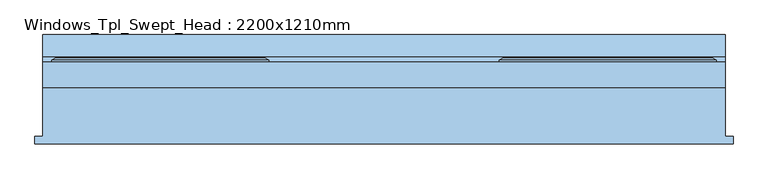
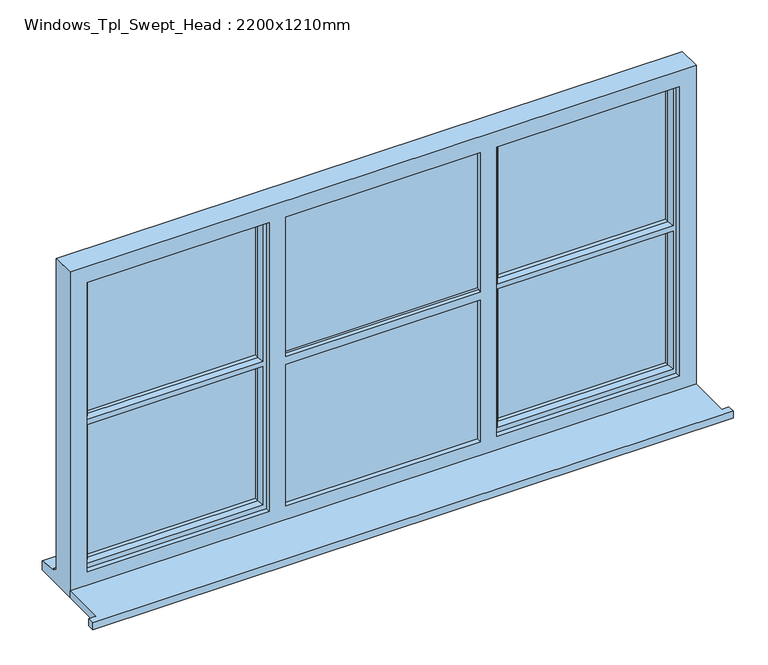
"""IFC4 building model written with IfcOpenShell, lengths in millimetres: window geometry, Windows_Tpl_Swept_Head : 2200x1210mm."""

from ifc_helpers import new_model, si_unit, point, frame, frame_2d, origin, place, context, project, spatial, polyline, circle_curve, trimmed, segment, composite_curve, outline, extrude, faceted_brep, source, transform, mapped, element, save


def windows_tpl_swept_head_2200x1210mm_9d782c46(model_context):
    return source(origin(), model_context, "Body", "SolidModel", [
        extrude(outline(polyline([(-1766.6666667, -161.5434322), (-1766.6666667, -136.5434322), (-1741.6666667, -136.5434322), (-1741.6666667, 20.4565678), (458.3333333, 20.4565678), (458.3333333, -136.5434322), (483.3333333, -136.5434322), (483.3333333, -161.5434322), (-1766.6666667, -161.5434322)])), frame((0.0, 0.0, 900.0), z_axis=(0.0, 0.0, 1.0), x_axis=(1.0, 0.0, 0.0)), (0.0, 0.0, 1.0), 25.0),
        extrude(outline(composite_curve([segment(polyline([(2050.0, -300.0), (2050.0, -983.3333333), (1935.9532624, -983.3333333)]), True, "CONTINUOUS"), segment(trimmed(circle_curve(frame_2d((1325.0, -641.6666667)), 700.0), [point((1935.9532624, -983.3333333))], [point((1935.9532624, -300.0))], True, "CARTESIAN"), True, "CONTINUOUS"), segment(polyline([(1935.9532624, -300.0), (2050.0, -300.0)]), True, "CONTINUOUS")], self_intersect=False)), frame((0.0, 62.4565678, 0.0), z_axis=(0.0, 1.0, 0.0), x_axis=(0.0, 0.0, 1.0)), (0.0, 0.0, 1.0), 25.0),
        extrude(outline(composite_curve([segment(polyline([(2030.0, -220.0), (1957.8501446, -220.0)]), True, "CONTINUOUS"), segment(trimmed(circle_curve(frame_2d((1325.0, 79.1666667)), 700.0), [point((1957.8501446, -220.0))], [point((1957.8501446, 378.3333333))], True, "CARTESIAN"), True, "CONTINUOUS"), segment(polyline([(1957.8501446, 378.3333333), (2030.0, 378.3333333), (2030.0, -220.0)]), True, "CONTINUOUS")], self_intersect=False)), frame((0.0, 79.4565678, 0.0), z_axis=(0.0, 1.0, 0.0), x_axis=(0.0, 0.0, 1.0)), (0.0, 0.0, 1.0), 24.0),
        extrude(outline(composite_curve([segment(polyline([(2030.0, -1063.3333333), (2030.0, -1661.6666667), (1957.8501446, -1661.6666667)]), True, "CONTINUOUS"), segment(trimmed(circle_curve(frame_2d((1325.0, -1362.5)), 700.0), [point((1957.8501446, -1661.6666667))], [point((1957.8501446, -1063.3333333))], True, "CARTESIAN"), True, "CONTINUOUS"), segment(polyline([(1957.8501446, -1063.3333333), (2030.0, -1063.3333333)]), True, "CONTINUOUS")], self_intersect=False)), frame((0.0, 79.4565678, 0.0), z_axis=(0.0, 1.0, 0.0), x_axis=(0.0, 0.0, 1.0)), (0.0, 0.0, 1.0), 24.0),
        faceted_brep([(-270.0, 103.4565678, 2080.0), (-270.0, 109.2300705, 2080.0), (-270.0, 109.2300705, 953.0), (-270.0, 103.4565678, 953.0), (-260.0, 38.4565678, 2070.0), (-260.0, 103.4565678, 2070.0), (-260.0, 103.4565678, 963.0), (-260.0, 38.4565678, 963.0), (-220.0, 52.9494677, 2030.0), (-230.1480377, 38.4565678, 2040.1480377), (-230.1480377, 38.4565678, 1526.3519623), (-220.0, 52.9494677, 1536.5), (-230.1480377, 38.4565678, 992.8519623), (-220.0, 52.9494677, 1003.0), (-220.0, 52.9494677, 1496.5), (-230.1480377, 38.4565678, 1506.6480377), (-220.0, 67.4565678, 2030.0), (-220.0, 67.4565678, 1536.5), (-220.0, 67.4565678, 1003.0), (-220.0, 67.4565678, 1496.5), (-230.0, 91.4565678, 1529.5), (-230.0, 91.4565678, 2040.0), (-230.0, 67.4565678, 2040.0), (-230.0, 67.4565678, 1529.5), (-230.0, 67.4565678, 1503.5), (-230.0, 67.4565678, 993.0), (-230.0, 91.4565678, 993.0), (-230.0, 91.4565678, 1503.5), (-220.0, 109.2300705, 2030.0), (-220.0, 91.4565678, 2030.0), (-220.0, 91.4565678, 1536.5), (-220.0, 109.2300705, 1536.5), (-220.0, 91.4565678, 1003.0), (-220.0, 109.2300705, 1003.0), (-220.0, 109.2300705, 1496.5), (-220.0, 91.4565678, 1496.5), (-237.4457548, 115.0035732, 2047.4457548), (-237.4457548, 115.0035732, 1519.0542452), (-237.4457548, 115.0035732, 985.5542452), (-237.4457548, 115.0035732, 1513.9457548), (-259.2153903, 115.0035732, 2069.2153903), (-259.2153903, 115.0035732, 963.7846097), (428.3333333, 109.2300705, 953.0), (428.3333333, 103.4565678, 953.0), (418.3333333, 103.4565678, 963.0), (418.3333333, 38.4565678, 963.0), (388.4813711, 38.4565678, 992.8519623), (378.3333333, 52.9494677, 1003.0), (378.3333333, 67.4565678, 1003.0), (388.3333333, 67.4565678, 993.0), (388.3333333, 91.4565678, 993.0), (378.3333333, 91.4565678, 1003.0), (378.3333333, 109.2300705, 1003.0), (395.7790881, 115.0035732, 985.5542452), (417.5487236, 115.0035732, 963.7846097), (428.3333333, 109.2300705, 2080.0), (428.3333333, 103.4565678, 2080.0), (418.3333333, 103.4565678, 2070.0), (418.3333333, 38.4565678, 2070.0), (388.4813711, 38.4565678, 1506.6480377), (378.3333333, 52.9494677, 1496.5), (388.4813711, 38.4565678, 2040.1480377), (378.3333333, 52.9494677, 2030.0), (378.3333333, 52.9494677, 1536.5), (388.4813711, 38.4565678, 1526.3519623), (378.3333333, 67.4565678, 1496.5), (378.3333333, 67.4565678, 2030.0), (378.3333333, 67.4565678, 1536.5), (388.3333333, 91.4565678, 1503.5), (388.3333333, 67.4565678, 1503.5), (388.3333333, 67.4565678, 1529.5), (388.3333333, 67.4565678, 2040.0), (388.3333333, 91.4565678, 2040.0), (388.3333333, 91.4565678, 1529.5), (378.3333333, 91.4565678, 1496.5), (378.3333333, 109.2300705, 1496.5), (378.3333333, 91.4565678, 2030.0), (378.3333333, 109.2300705, 2030.0), (378.3333333, 109.2300705, 1536.5), (378.3333333, 91.4565678, 1536.5), (395.7790881, 115.0035732, 1513.9457548), (395.7790881, 115.0035732, 2047.4457548), (395.7790881, 115.0035732, 1519.0542452), (417.5487236, 115.0035732, 2069.2153903)], [[[0, 1, 2, 3]], [[4, 5, 6, 7]], [[8, 9, 10, 11]], [[12, 13, 14, 15]], [[16, 8, 11, 17]], [[13, 18, 19, 14]], [[20, 21, 22, 23]], [[24, 25, 26, 27]], [[28, 29, 30, 31]], [[32, 33, 34, 35]], [[36, 28, 31, 37]], [[33, 38, 39, 34]], [[2, 1, 40, 41]], [[3, 2, 42, 43]], [[7, 6, 44, 45]], [[13, 12, 46, 47]], [[18, 13, 47, 48]], [[26, 25, 49, 50]], [[33, 32, 51, 52]], [[38, 33, 52, 53]], [[2, 41, 54, 42]], [[43, 42, 55, 56]], [[45, 44, 57, 58]], [[47, 46, 59, 60]], [[61, 62, 63, 64]], [[48, 47, 60, 65]], [[62, 66, 67, 63]], [[68, 50, 49, 69]], [[70, 71, 72, 73]], [[52, 51, 74, 75]], [[76, 77, 78, 79]], [[53, 52, 75, 80]], [[77, 81, 82, 78]], [[42, 54, 83, 55]], [[1, 0, 56, 55]], [[0, 3, 43, 56], [6, 5, 57, 44]], [[5, 4, 58, 57]], [[4, 7, 45, 58], [46, 12, 15, 59], [61, 64, 10, 9]], [[9, 8, 62, 61]], [[8, 16, 66, 62]], [[49, 25, 24, 69], [18, 48, 65, 19]], [[22, 71, 70, 23], [66, 16, 17, 67]], [[22, 21, 72, 71]], [[26, 50, 68, 27], [32, 35, 74, 51]], [[72, 21, 20, 73], [76, 79, 30, 29]], [[29, 28, 77, 76]], [[28, 36, 81, 77]], [[41, 40, 83, 54], [36, 37, 82, 81], [38, 53, 80, 39]], [[40, 1, 55, 83]], [[82, 37, 31, 78]], [[30, 79, 78, 31]], [[73, 20, 23, 70]], [[11, 63, 67, 17]], [[10, 64, 63, 11]], [[59, 15, 14, 60]], [[60, 14, 19, 65]], [[27, 68, 69, 24]], [[74, 35, 34, 75]], [[39, 80, 75, 34]]]),
        faceted_brep([(-1013.3333333, 103.4565678, 2080.0), (-1013.3333333, 109.2300705, 2080.0), (-1711.6666667, 109.2300705, 2080.0), (-1711.6666667, 103.4565678, 2080.0), (-1023.3333333, 38.4565678, 2070.0), (-1023.3333333, 103.4565678, 2070.0), (-1701.6666667, 103.4565678, 2070.0), (-1701.6666667, 38.4565678, 2070.0), (-1063.3333333, 52.9494677, 2030.0), (-1053.1852956, 38.4565678, 2040.1480377), (-1671.8147044, 38.4565678, 2040.1480377), (-1661.6666667, 52.9494677, 2030.0), (-1661.6666667, 67.4565678, 2030.0), (-1063.3333333, 67.4565678, 2030.0), (-1053.3333333, 91.4565678, 2040.0), (-1053.3333333, 67.4565678, 2040.0), (-1671.6666667, 67.4565678, 2040.0), (-1671.6666667, 91.4565678, 2040.0), (-1063.3333333, 109.2300705, 2030.0), (-1063.3333333, 91.4565678, 2030.0), (-1661.6666667, 91.4565678, 2030.0), (-1661.6666667, 109.2300705, 2030.0), (-1679.1124215, 115.0035732, 2047.4457548), (-1045.8875785, 115.0035732, 2047.4457548), (-1024.117943, 115.0035732, 2069.2153903), (-1700.882057, 115.0035732, 2069.2153903), (-1711.6666667, 109.2300705, 953.0), (-1711.6666667, 103.4565678, 953.0), (-1701.6666667, 103.4565678, 963.0), (-1701.6666667, 38.4565678, 963.0), (-1671.8147044, 38.4565678, 1526.3519623), (-1661.6666667, 52.9494677, 1536.5), (-1671.8147044, 38.4565678, 992.8519623), (-1661.6666667, 52.9494677, 1003.0), (-1661.6666667, 52.9494677, 1496.5), (-1671.8147044, 38.4565678, 1506.6480377), (-1661.6666667, 67.4565678, 1536.5), (-1661.6666667, 67.4565678, 1003.0), (-1661.6666667, 67.4565678, 1496.5), (-1671.6666667, 91.4565678, 1529.5), (-1671.6666667, 67.4565678, 1529.5), (-1671.6666667, 67.4565678, 1503.5), (-1671.6666667, 67.4565678, 993.0), (-1671.6666667, 91.4565678, 993.0), (-1671.6666667, 91.4565678, 1503.5), (-1661.6666667, 91.4565678, 1536.5), (-1661.6666667, 109.2300705, 1536.5), (-1661.6666667, 91.4565678, 1003.0), (-1661.6666667, 109.2300705, 1003.0), (-1661.6666667, 109.2300705, 1496.5), (-1661.6666667, 91.4565678, 1496.5), (-1679.1124215, 115.0035732, 1519.0542452), (-1679.1124215, 115.0035732, 985.5542452), (-1679.1124215, 115.0035732, 1513.9457548), (-1700.882057, 115.0035732, 963.7846097), (-1013.3333333, 109.2300705, 953.0), (-1013.3333333, 103.4565678, 953.0), (-1023.3333333, 103.4565678, 963.0), (-1023.3333333, 38.4565678, 963.0), (-1053.1852956, 38.4565678, 1526.3519623), (-1053.1852956, 38.4565678, 1506.6480377), (-1053.1852956, 38.4565678, 992.8519623), (-1063.3333333, 52.9494677, 1003.0), (-1063.3333333, 67.4565678, 1003.0), (-1053.3333333, 67.4565678, 1529.5), (-1063.3333333, 67.4565678, 1536.5), (-1053.3333333, 67.4565678, 993.0), (-1053.3333333, 67.4565678, 1503.5), (-1063.3333333, 67.4565678, 1496.5), (-1053.3333333, 91.4565678, 993.0), (-1053.3333333, 91.4565678, 1529.5), (-1063.3333333, 91.4565678, 1536.5), (-1053.3333333, 91.4565678, 1503.5), (-1063.3333333, 91.4565678, 1496.5), (-1063.3333333, 91.4565678, 1003.0), (-1063.3333333, 109.2300705, 1003.0), (-1045.8875785, 115.0035732, 985.5542452), (-1024.117943, 115.0035732, 963.7846097), (-1045.8875785, 115.0035732, 1519.0542452), (-1045.8875785, 115.0035732, 1513.9457548), (-1063.3333333, 52.9494677, 1536.5), (-1063.3333333, 52.9494677, 1496.5), (-1063.3333333, 109.2300705, 1536.5), (-1063.3333333, 109.2300705, 1496.5)], [[[0, 1, 2, 3]], [[4, 5, 6, 7]], [[8, 9, 10, 11]], [[8, 11, 12, 13]], [[14, 15, 16, 17]], [[18, 19, 20, 21]], [[18, 21, 22, 23]], [[2, 1, 24, 25]], [[3, 2, 26, 27]], [[7, 6, 28, 29]], [[11, 10, 30, 31]], [[32, 33, 34, 35]], [[12, 11, 31, 36]], [[33, 37, 38, 34]], [[39, 17, 16, 40]], [[41, 42, 43, 44]], [[21, 20, 45, 46]], [[47, 48, 49, 50]], [[22, 21, 46, 51]], [[48, 52, 53, 49]], [[2, 25, 54, 26]], [[27, 26, 55, 56]], [[0, 3, 27, 56], [6, 5, 57, 28]], [[29, 28, 57, 58]], [[4, 7, 29, 58], [10, 9, 59, 30], [32, 35, 60, 61]], [[33, 32, 61, 62]], [[37, 33, 62, 63]], [[16, 15, 64, 40], [13, 12, 36, 65]], [[66, 42, 41, 67], [37, 63, 68, 38]], [[43, 42, 66, 69]], [[14, 17, 39, 70], [19, 71, 45, 20]], [[43, 69, 72, 44], [47, 50, 73, 74]], [[48, 47, 74, 75]], [[52, 48, 75, 76]], [[25, 24, 77, 54], [23, 22, 51, 78], [76, 79, 53, 52]], [[26, 54, 77, 55]], [[1, 0, 56, 55]], [[5, 4, 58, 57]], [[9, 8, 80, 59]], [[62, 61, 60, 81]], [[8, 13, 65, 80]], [[63, 62, 81, 68]], [[64, 15, 14, 70]], [[72, 69, 66, 67]], [[19, 18, 82, 71]], [[75, 74, 73, 83]], [[18, 23, 78, 82]], [[76, 75, 83, 79]], [[24, 1, 55, 77]], [[78, 51, 46, 82]], [[45, 71, 82, 46]], [[40, 64, 70, 39]], [[65, 36, 31, 80]], [[30, 59, 80, 31]], [[60, 35, 34, 81]], [[38, 68, 81, 34]], [[67, 41, 44, 72]], [[73, 50, 49, 83]], [[53, 79, 83, 49]]]),
        extrude(outline(polyline([(388.4813711, 67.4565678), (-230.0, 67.4565678), (-230.0, 91.4565678), (388.4813711, 91.4565678), (388.4813711, 67.4565678)])), frame((0.0, 0.0, 993.0), z_axis=(0.0, 0.0, 1.0), x_axis=(1.0, 0.0, 0.0)), (0.0, 0.0, 1.0), 513.6480377),
        extrude(outline(polyline([(388.4813711, 67.4565678), (-230.0, 67.4565678), (-230.0, 91.4565678), (388.4813711, 91.4565678), (388.4813711, 67.4565678)])), frame((0.0, 0.0, 1526.3519623), z_axis=(0.0, 0.0, 1.0), x_axis=(1.0, 0.0, 0.0)), (0.0, 0.0, 1.0), 513.6480377),
        extrude(outline(polyline([(-993.3333333, 62.4565678), (-290.0, 62.4565678), (-290.0, 38.4565678), (-993.3333333, 38.4565678), (-993.3333333, 62.4565678)])), frame((0.0, 0.0, 963.0), z_axis=(0.0, 0.0, 1.0), x_axis=(1.0, 0.0, 0.0)), (0.0, 0.0, 1.0), 540.5),
        extrude(outline(polyline([(-993.3333333, 62.4565678), (-290.0, 62.4565678), (-290.0, 38.4565678), (-993.3333333, 38.4565678), (-993.3333333, 62.4565678)])), frame((0.0, 0.0, 1529.5), z_axis=(0.0, 0.0, 1.0), x_axis=(1.0, 0.0, 0.0)), (0.0, 0.0, 1.0), 540.5),
        extrude(outline(polyline([(-1053.3333333, 67.4565678), (-1671.6666667, 67.4565678), (-1671.6666667, 91.4565678), (-1053.3333333, 91.4565678), (-1053.3333333, 67.4565678)])), frame((0.0, 0.0, 1526.3519623), z_axis=(0.0, 0.0, 1.0), x_axis=(1.0, 0.0, 0.0)), (0.0, 0.0, 1.0), 513.6480377),
        extrude(outline(polyline([(-1053.3333333, 67.4565678), (-1671.6666667, 67.4565678), (-1671.6666667, 91.4565678), (-1053.3333333, 91.4565678), (-1053.3333333, 67.4565678)])), frame((0.0, 0.0, 993.0), z_axis=(0.0, 0.0, 1.0), x_axis=(1.0, 0.0, 0.0)), (0.0, 0.0, 1.0), 513.6480377),
        faceted_brep([(-983.3333333, 38.4565678, 2050.0), (-983.3333333, 20.4565678, 2050.0), (-983.3333333, 20.4565678, 1530.8390708), (-983.3333333, 28.5412125, 1536.5), (-983.3333333, 38.4565678, 1536.5), (-983.3333333, 20.4565678, 975.0), (-983.3333333, 38.4565678, 975.0), (-983.3333333, 38.4565678, 1496.5), (-983.3333333, 28.5412125, 1496.5), (-983.3333333, 20.4565678, 1502.1609292), (458.3333333, 20.4565678, 2110.0), (-1741.6666667, 20.4565678, 2110.0), (-1741.6666667, 20.4565678, 900.0), (458.3333333, 20.4565678, 900.0), (-1681.6666667, 20.4565678, 2050.0), (-1041.3333333, 20.4565678, 2050.0), (-1041.3333333, 20.4565678, 975.0), (-1681.6666667, 20.4565678, 975.0), (-242.0, 20.4565678, 2050.0), (398.3333333, 20.4565678, 2050.0), (398.3333333, 20.4565678, 975.0), (-242.0, 20.4565678, 975.0), (-300.0, 20.4565678, 2050.0), (-300.0, 20.4565678, 1530.8390708), (-300.0, 20.4565678, 975.0), (-300.0, 20.4565678, 1502.1609292), (-1041.3333333, 38.4565678, 2050.0), (-1041.3333333, 38.4565678, 975.0), (-1701.6666667, 38.4565678, 2070.0), (-1023.3333333, 38.4565678, 2070.0), (-1023.3333333, 38.4565678, 963.0), (-1701.6666667, 38.4565678, 963.0), (-1681.6666667, 38.4565678, 2050.0), (-1681.6666667, 38.4565678, 975.0), (-993.3333333, 38.4565678, 2070.0), (-290.0, 38.4565678, 2070.0), (-290.0, 38.4565678, 1529.5), (-983.3333333, 38.4565678, 1529.5), (-983.3333333, 38.4565678, 1503.5), (-290.0, 38.4565678, 1503.5), (-290.0, 38.4565678, 963.0), (-993.3333333, 38.4565678, 963.0), (-300.0, 38.4565678, 2050.0), (-300.0, 38.4565678, 1536.5), (-300.0, 38.4565678, 975.0), (-300.0, 38.4565678, 1496.5), (-260.0, 38.4565678, 2070.0), (418.3333333, 38.4565678, 2070.0), (418.3333333, 38.4565678, 963.0), (-260.0, 38.4565678, 963.0), (398.3333333, 38.4565678, 2050.0), (-242.0, 38.4565678, 2050.0), (-242.0, 38.4565678, 975.0), (398.3333333, 38.4565678, 975.0), (-1023.3333333, 103.4565678, 2070.0), (-1023.3333333, 103.4565678, 963.0), (-1741.6666667, 103.4565678, 2110.0), (458.3333333, 103.4565678, 2110.0), (458.3333333, 103.4565678, 951.0), (-1741.6666667, 103.4565678, 951.0), (-1701.6666667, 103.4565678, 2070.0), (-1701.6666667, 103.4565678, 963.0), (-983.3333333, 103.4565678, 2070.0), (-983.3333333, 103.4565678, 963.0), (-300.0, 103.4565678, 963.0), (-300.0, 103.4565678, 2070.0), (418.3333333, 103.4565678, 963.0), (418.3333333, 103.4565678, 2070.0), (-260.0, 103.4565678, 2070.0), (-260.0, 103.4565678, 963.0), (-983.3333333, 98.4565678, 2070.0), (-983.3333333, 98.4565678, 2050.0), (-983.3333333, 62.4565678, 2050.0), (-983.3333333, 62.4565678, 1536.5), (-983.3333333, 80.2300705, 1536.5), (-983.3333333, 86.0035732, 1519.0542452), (-983.3333333, 86.0035732, 1513.9457548), (-983.3333333, 80.2300705, 1496.5), (-983.3333333, 62.4565678, 1496.5), (-983.3333333, 62.4565678, 975.0), (-983.3333333, 98.4565678, 975.0), (-983.3333333, 98.4565678, 963.0), (-290.0, 62.4565678, 1503.5), (-983.3333333, 62.4565678, 1503.5), (-983.3333333, 62.4565678, 1529.5), (-290.0, 62.4565678, 1529.5), (-290.0, 62.4565678, 2070.0), (-993.3333333, 62.4565678, 2070.0), (-993.3333333, 62.4565678, 963.0), (-290.0, 62.4565678, 963.0), (-300.0, 62.4565678, 2050.0), (-300.0, 62.4565678, 1536.5), (-300.0, 62.4565678, 1496.5), (-300.0, 62.4565678, 975.0), (-1741.6666667, 118.4565678, 949.68767), (-1741.6666667, 118.4565678, 944.7449676), (-1741.6666667, 190.9565678, 933.8088847), (-1741.6666667, 190.9565678, 900.0), (-300.0, 98.4565678, 2070.0), (458.3333333, 190.9565678, 900.0), (458.3333333, 190.9565678, 933.8088847), (458.3333333, 118.4565678, 944.7449676), (458.3333333, 118.4565678, 949.68767), (-300.0, 98.4565678, 963.0), (-300.0, 98.4565678, 975.0), (-300.0, 80.2300705, 1496.5), (-300.0, 86.0035732, 1513.9457548), (-300.0, 86.0035732, 1519.0542452), (-300.0, 80.2300705, 1536.5), (-300.0, 98.4565678, 2050.0), (-300.0, 28.5412125, 1536.5), (-300.0, 28.5412125, 1496.5)], [[[0, 1, 2, 3, 4]], [[5, 6, 7, 8, 9]], [[10, 11, 12, 13], [14, 15, 16, 17], [18, 19, 20, 21], [1, 22, 23, 2], [24, 5, 9, 25]], [[15, 26, 27, 16]], [[28, 29, 30, 31], [26, 32, 33, 27]], [[34, 35, 36, 37, 38, 39, 40, 41], [42, 0, 4, 43], [6, 44, 45, 7]], [[46, 47, 48, 49], [50, 51, 52, 53]], [[54, 55, 30, 29]], [[56, 57, 58, 59], [55, 54, 60, 61], [62, 63, 64, 65], [66, 67, 68, 69]], [[63, 62, 70, 71, 72, 73, 74, 75, 76, 77, 78, 79, 80, 81]], [[82, 83, 84, 85, 86, 87, 88, 89], [73, 72, 90, 91], [92, 93, 79, 78]], [[88, 87, 34, 41]], [[11, 56, 59, 94, 95, 96, 97, 12]], [[61, 60, 28, 31]], [[32, 14, 17, 33]], [[11, 10, 57, 56]], [[62, 65, 98, 70]], [[87, 86, 35, 34]], [[28, 60, 54, 29]], [[67, 47, 46, 68]], [[1, 0, 42, 22]], [[14, 32, 26, 15]], [[50, 19, 18, 51]], [[57, 10, 13, 99, 100, 101, 102, 58]], [[67, 66, 48, 47]], [[19, 50, 53, 20]], [[82, 89, 40, 39]], [[35, 86, 85, 36]], [[65, 64, 103, 104, 93, 92, 105, 106, 107, 108, 91, 90, 109, 98]], [[69, 68, 46, 49]], [[51, 18, 21, 52]], [[22, 42, 43, 110, 23]], [[44, 24, 25, 111, 45]], [[99, 13, 12, 97]], [[100, 99, 97, 96]], [[101, 100, 96, 95]], [[102, 101, 95, 94]], [[58, 102, 94, 59]], [[55, 61, 31, 30]], [[64, 63, 81, 103]], [[66, 69, 49, 48]], [[89, 88, 41, 40]], [[17, 16, 27, 33]], [[21, 20, 53, 52]], [[44, 6, 5, 24]], [[83, 38, 37, 84]], [[75, 107, 106, 76]], [[76, 106, 105, 77]], [[92, 78, 77, 105]], [[38, 83, 82, 39]], [[7, 45, 111, 8]], [[25, 9, 8, 111]], [[2, 23, 110, 3]], [[43, 4, 3, 110]], [[84, 37, 36, 85]], [[73, 91, 108, 74]], [[107, 75, 74, 108]], [[79, 93, 104, 80]], [[80, 104, 103, 81]], [[109, 71, 70, 98]], [[90, 72, 71, 109]]]),
    ])


if __name__ == "__main__":
    model = new_model("IFC4")
    model_context = context("Model", 3, world=origin())
    ifc_project = project(units=[si_unit("LENGTHUNIT", "METRE", prefix="MILLI")], contexts=[model_context])
    site = spatial("IfcSite", under=ifc_project)
    building = spatial("IfcBuilding", under=site)
    placement = place(None, origin())
    windows_tpl_swept_head_2200x1210mm_shape = windows_tpl_swept_head_2200x1210mm_9d782c46(model_context)
    element("IfcWindow", 1, ObjectType="Windows_Tpl_Swept_Head : 2200x1210mm", at=placement, inside=building, context=model_context, shape_type="MappedRepresentation", body=[
        mapped(windows_tpl_swept_head_2200x1210mm_shape, transform((0.0, 0.0, 0.0), x_axis=(1.0, 0.0, 0.0), y_axis=(0.0, 1.0, 0.0), z_axis=(0.0, 0.0, 1.0))),
    ])
    save(model, "model.ifc")

# Revit data of these elements
# Type "Windows_Tpl_Swept_Head : 2200x1210mm"
#   Type Mark = "57"
#   Operation = "TriplePanelVertical"
#   Construction Type Id = "GSP4R"
#   Manufacturer = "Revit"
#   Keynote = "L10"
#   Analytic Construction = "1/8 in Pilkington single glazing"
#   Wrap Layers (Ext) from Ext = 102.5 mm
#   Wrap Layers (Int) from Ext = 177.5 mm
#   Window Board Projection = 25 mm
#   Window Board Extension = 25 mm
#   Visual Light Transmittance = 0.9
#   Solar Heat Gain Coefficient = 0.78
#   Rough Width = 2200 mm
#   Rough Height = 1210 mm
#   Radius - Swept Head = 700 mm
#   Height = 1210 mm
#   Width = 2200 mm
#   Heat Transfer Coefficient (U) = 3.6886 W/(m²·K)
#   Glazing Thickness = 24 mm
#   FrameOffset - External = 50 mm
#   Frame Depth = 65 mm
#   Default Head Height = 2110 mm
#   Cill Depth = 87.5 mm
#   Cavity Closer Width = 50 mm
#   Cavity Closer Offset from Ext = 102.5 mm
#   Cavity Closer Depth = 85 mm
#   Vis - Cavity Closers = yes
#   Material Trim = Window Frame
#   Material Glass = Glass
#   Material Frame = Window Frame
#   Wall Closure = (empty or 0)
# Element 1 (IfcWindow, "Windows_Tpl_Swept_Head : 2200x1210mm")
#   Materials on its faces: "Window Frame", "Glass"
# Materials
#   "Window Frame": class "Miscellaneous", colour RGB 249 249 249, transparency 0, Keynote = "L10", Cost = 0
#   "Glass": class "Glass", colour RGB 0 128 192, transparency 0.9, Description = "Soda Lime Glass", Cost = 0
